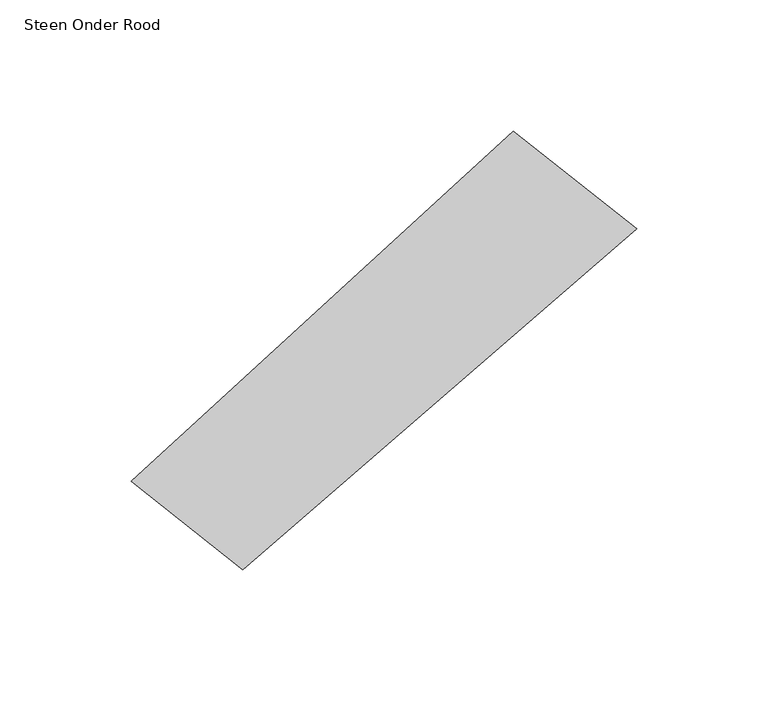
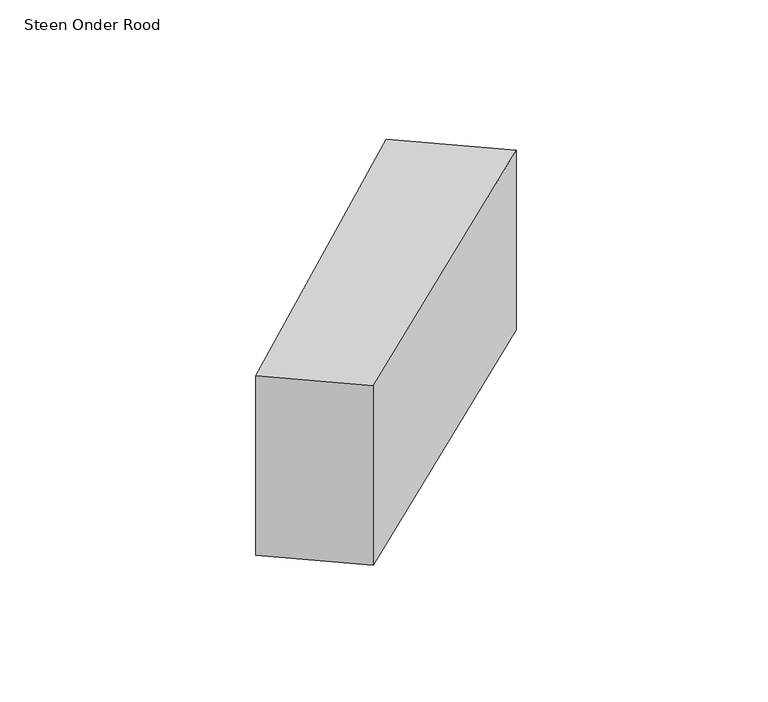
"""IFC4 building model written with IfcOpenShell, lengths in millimetres: proxy geometry, 00_GMA_steen_versie_4 : Steen Onder Rood."""

from ifc_helpers import new_model, si_unit, origin, origin_with_axes, place, context, project, spatial, polyline, outline, extrude, source, transform, mapped, element, save


def steen_onder_rood_ccd546c7(model_context):
    return source(origin(), model_context, "Body", "SweptSolid", [
        extrude(outline(polyline([(184.3134395, 84.9677266), (34.0851218, -44.8937007), (-8.4749227, -11.1599186), (137.2682622, 122.2297146), (184.3134395, 84.9677266)])), origin_with_axes(), (0.0, 0.0, 1.0), 100.0),
    ])


if __name__ == "__main__":
    model = new_model("IFC4")
    model_context = context("Model", 3, world=origin())
    ifc_project = project(units=[si_unit("LENGTHUNIT", "METRE", prefix="MILLI")], contexts=[model_context])
    site = spatial("IfcSite", under=ifc_project)
    building = spatial("IfcBuilding", under=site)
    placement = place(None, origin())
    steen_onder_rood_shape = steen_onder_rood_ccd546c7(model_context)
    element("IfcBuildingElementProxy", 1, Name="00_GMA_steen_versie_4 : Steen Onder Rood", ObjectType="00_GMA_steen_versie_4 : Steen Onder Rood", at=placement, inside=building, context=model_context, shape_type="MappedRepresentation", body=[
        mapped(steen_onder_rood_shape, transform((0.0, 0.0, 0.0), x_axis=(1.0, 0.0, 0.0), y_axis=(0.0, 1.0, 0.0), z_axis=(0.0, 0.0, 1.0))),
    ])
    save(model, "model.ifc")

# Revit data of these elements
# Type "00_GMA_steen_versie_4 : Steen Onder Rood"
#   StootVoegHalfBoven [instance default] = 5 mm
#   StootVoegHalf [instance default] = 5 mm
#   StootVoegBreedteOnder = 10 mm
#   StootVoegBreedteBoven = 10 mm
#   Steendikte = 100 mm
#   LintVoegOnderHalf = 0 mm
#   LintVoegOnder = 0 mm
#   LintVoegBovenHalf = 5 mm
#   LintVoegBoven = 10 mm
#   materiaal = 21_steen_rood
#   MateriaalVoeg = none
#   Default Elevation = 0
# Element 1 (IfcBuildingElementProxy, "00_GMA_steen_versie_4 : Steen Onder Rood")
#   Materials on its faces: "21_steen_rood"
# Materials
#   "21_steen_rood": class "Unassigned", colour RGB 213 111 43, transparency 0, Cost = 0
